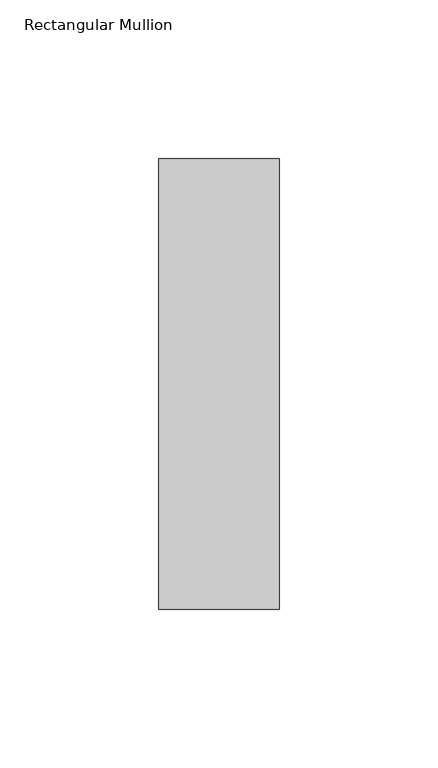
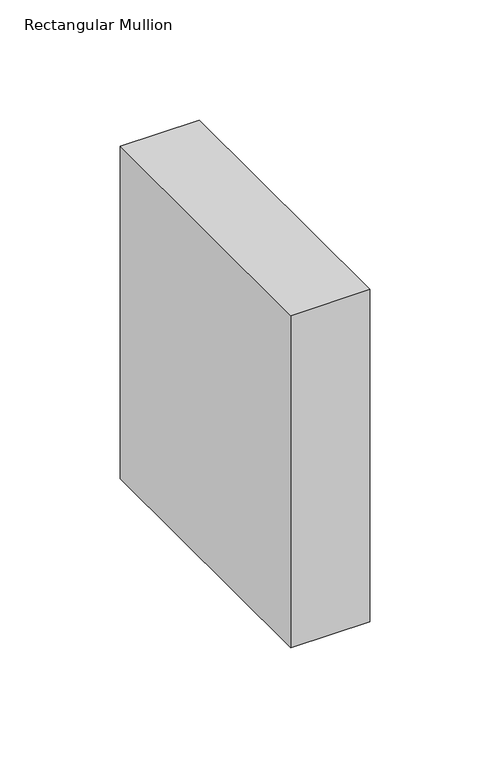
"""IFC4 building model written with IfcOpenShell, lengths in millimetres: member geometry, Rectangular Mullion : NLRS_21_CWM_hsb-regel 38x142_gen_rsf."""

from ifc_helpers import new_model, si_unit, frame, origin, place, context, project, spatial, polyline, outline, extrude, source, transform, mapped, element, save


def rectangular_mullion_1f17af45(model_context):
    return source(origin(), model_context, "Body", "SweptSolid", [
        extrude(outline(polyline([(0.0, -71.0), (-38.0, -71.0), (-38.0, 71.0), (0.0, 71.0), (0.0, -71.0)])), frame((0.0, 0.0, -168.9999997), z_axis=(0.0, 0.0, 1.0), x_axis=(1.0, 0.0, 0.0)), (0.0, 0.0, 1.0), 168.9999997),
    ])


if __name__ == "__main__":
    model = new_model("IFC4")
    model_context = context("Model", 3, world=origin())
    ifc_project = project(units=[si_unit("LENGTHUNIT", "METRE", prefix="MILLI")], contexts=[model_context])
    site = spatial("IfcSite", under=ifc_project)
    building = spatial("IfcBuilding", under=site)
    placement = place(None, origin())
    rectangular_mullion_shape = rectangular_mullion_1f17af45(model_context)
    element("IfcMember", 1, ObjectType="Rectangular Mullion : NLRS_21_CWM_hsb-regel 38x142_gen_rsf", at=placement, inside=building, context=model_context, shape_type="MappedRepresentation", body=[
        mapped(rectangular_mullion_shape, transform((0.0, 0.0, 0.0), x_axis=(1.0, 0.0, 0.0), y_axis=(0.0, 1.0, 0.0), z_axis=(0.0, 0.0, 1.0))),
    ])
    save(model, "model.ifc")

# Revit data of these elements
# Type "Rectangular Mullion : NLRS_21_CWM_hsb-regel 38x142_gen_rsf"
#   Export Type to IFC As = "IfcWall"
#   Type IfcGUID = "07M7mRoiH1CR8m_RSKIwpF"
#   Assembly Code = "21.10"
#   built-in parameter 1007322 = 0.465879 (stored number, unit not read)
#   built-in parameter 1007321 = 0.062336 (stored number, unit not read)
#   built-in parameter 1007320 = 0.062336 (stored number, unit not read)
# Element 1 (IfcMember, "Rectangular Mullion : NLRS_21_CWM_hsb-regel 38x142_gen_rsf")
#   Materials on its faces: "NLRS_i2_hout naaldhout vuren_gen_rsf"
# Materials
#   "NLRS_i2_hout naaldhout vuren_gen_rsf": class "I - Hout", colour RGB 234 199 147, transparency 0, Keynote = "i2", Manufacturer = "Revit Standards Foundation", URL = "www.revitstandards.org", Description = "hout vuren", Cost = 0
